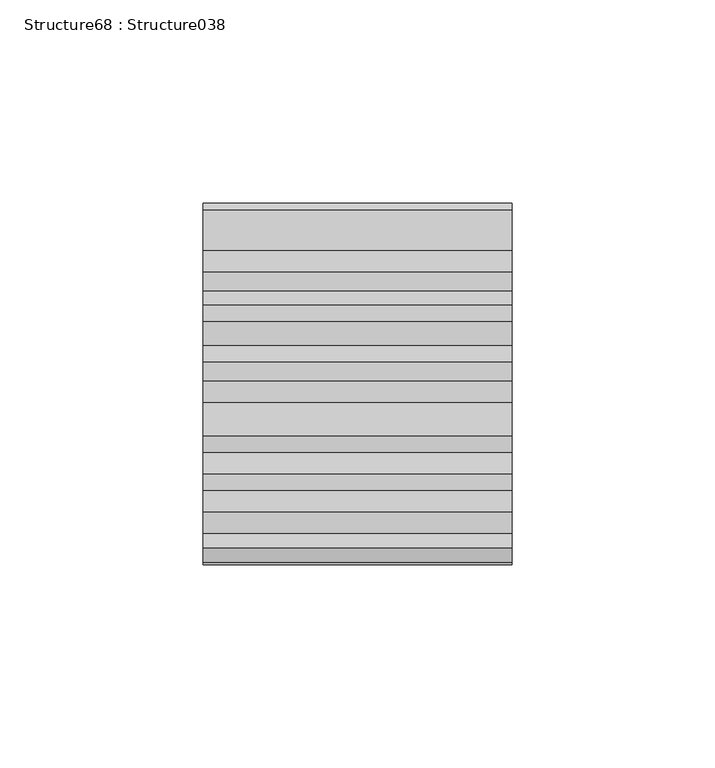
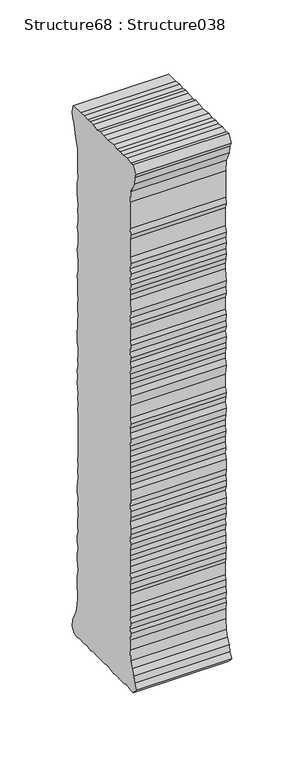
"""IFC4 building model written with IfcOpenShell, lengths in millimetres: proxy geometry, Structure68 : Structure038."""

from ifc_helpers import new_model, si_unit, frame, origin, place, context, project, spatial, polyline, outline, extrude, source, transform, mapped, element, save


def structure68_structure038_898fa140(model_context):
    return source(origin(), model_context, "Body", "SweptSolid", [
        extrude(outline(polyline([(279690.2824701, 3575.6853037), (279690.8761737, 3583.8864372), (279690.8761737, 3592.6700423), (279690.2824701, 3598.5284533), (279690.8761737, 3602.0280957), (279690.2824701, 3606.7295868), (279690.8761737, 3611.4134274), (279690.8761737, 3617.2718384), (279691.4586452, 3620.7971545), (279691.4586452, 3631.3410106), (279690.8761737, 3634.856699), (279690.8761737, 3640.114988), (279690.2824701, 3644.8245022), (279690.8761737, 3648.9258713), (279690.8761737, 3654.7842823), (279691.4586452, 3659.4584952), (279690.8761737, 3664.1423357), (279691.4586452, 3668.2437048), (279690.2824701, 3673.5276674), (279690.8761737, 3678.2018803), (279690.2824701, 3682.3289231), (279690.2824701, 3687.0127636), (279691.4586452, 3692.2710525), (279690.2824701, 3696.3884676), (279690.2824701, 3701.6547796), (279690.8761737, 3705.7545441), (279690.2824701, 3711.0304837), (279690.2824701, 3719.2316172), (279691.4586452, 3723.9154578), (279690.8761737, 3728.5992983), (279691.4586452, 3733.2991849), (279691.4586452, 3737.9750024), (279690.8761737, 3742.6748889), (279691.4586452, 3747.3587295), (279691.4586452, 3752.04257), (279690.8761737, 3756.7440611), (279690.2824701, 3762.5848215), (279691.4586452, 3767.2590344), (279690.8761737, 3771.9605256), (279690.2824701, 3775.4874463), (279691.4586452, 3780.1616592), (279691.4586452, 3790.7039107), (279690.2824701, 3798.9050443), (279691.4586452, 3804.1890069), (279691.4586452, 3808.8888934), (279690.8761737, 3813.5743386), (279690.8761737, 3817.6741031), (279690.2824701, 3822.932392), (279691.4586452, 3827.6162325), (279690.2824701, 3831.732043), (279690.8761737, 3836.4174882), (279690.2824701, 3842.2758992), (279691.4586452, 3845.8012153), (279691.4586452, 3855.7353217), (279690.2824701, 3859.8591552), (279690.8761737, 3865.1190488), (279690.2824701, 3870.4030114), (279691.4586452, 3879.7610648), (279691.4586452, 3884.4609514), (279690.8761737, 3888.5623205), (279690.2824701, 3893.246161), (279690.8761737, 3897.3475301), (279690.2824701, 3902.6314927), (279690.8761737, 3906.7328618), (279690.2824701, 3911.4054701), (279691.4586452, 3916.0909152), (279691.4586452, 3931.3346579), (279690.2824701, 3935.4328178), (279690.8761737, 3940.718385), (279690.8761737, 3962.9774586), (279690.2824701, 3972.3627903), (279685.6098618, 3981.7208437), (279685.0161581, 3987.5792547), (279683.2575116, 3991.0788971), (279686.765177, 3997.5486624), (279690.2824701, 3996.390138), (279695.5584096, 3997.5486624), (279700.8359538, 3996.9645864), (279704.9341137, 3997.5486624), (279710.2116579, 3996.390138), (279714.3114224, 3997.5486624), (279722.5189744, 3996.390138), (279727.7852863, 3996.9645864), (279732.4787545, 3997.5486624), (279736.5801236, 3996.390138), (279742.4305116, 3997.5486624), (279746.5366945, 3997.5486624), (279750.0475691, 3996.9645864), (279754.7394327, 3997.5486624), (279760.0137676, 3996.9645864), (279769.9735477, 3996.9645864), (279771.7321943, 3991.0788971), (279770.5656468, 3986.4046842), (279768.7989772, 3982.3225704), (279768.2245288, 3978.2035506), (279766.4562547, 3972.3627903), (279764.1151367, 3964.1343784), (279764.1151367, 3944.8165449), (279763.5310607, 3939.5325823), (279764.6992128, 3935.4328178), (279764.6992128, 3925.4746423), (279764.1151367, 3921.3748778), (279763.5310607, 3916.6653636), (279764.1151367, 3911.4054701), (279763.5310607, 3907.888177), (279763.5310607, 3903.2059411), (279764.6992128, 3897.3475301), (279763.5310607, 3893.246161), (279763.5310607, 3883.8881076), (279764.6992128, 3878.5784713), (279764.1151367, 3874.5043805), (279763.5310607, 3869.2444869), (279763.5310607, 3861.0192843), (279764.6992128, 3856.3161885), (279764.1151367, 3851.6612309), (279764.1151367, 3841.0900965), (279763.5310607, 3836.9919366), (279764.1151367, 3832.8921721), (279764.1151367, 3828.2163546), (279763.5310607, 3822.932392), (279764.1151367, 3818.8310229), (279764.1151367, 3812.9726119), (279764.6992128, 3808.8888934), (279764.6992128, 3800.0876378), (279763.5310607, 3795.4037973), (279763.5310607, 3790.7039107), (279764.1151367, 3785.4456218), (279763.5310607, 3781.3282066), (279764.6992128, 3776.0618947), (279764.1151367, 3770.8036057), (279764.6992128, 3766.1021146), (279764.1151367, 3762.0023501), (279763.5310607, 3756.7440611), (279764.1151367, 3753.2171405), (279763.5310607, 3748.5429276), (279764.1151367, 3742.6748889), (279763.5310607, 3739.1592005), (279763.5310607, 3705.7545441), (279764.1151367, 3700.4705815), (279763.5310607, 3696.3884676), (279764.1151367, 3691.0868544), (279763.5310607, 3686.4030139), (279764.1151367, 3681.7271964), (279764.6992128, 3677.6274319), (279764.6992128, 3673.5276674), (279763.5310607, 3668.8261762), (279764.1151367, 3663.5598643), (279763.5310607, 3658.8840468), (279763.5310607, 3654.1841602), (279764.1151367, 3649.5003197), (279764.1151367, 3644.2420307), (279763.5310607, 3640.114988), (279764.6992128, 3636.0408972), (279764.6992128, 3631.3410106), (279763.5310607, 3626.6571701), (279764.6992128, 3620.7971545), (279764.6992128, 3616.69739), (279764.1151367, 3612.5976255), (279763.5310607, 3607.3393366), (279764.6992128, 3602.0280957), (279764.6992128, 3592.6700423), (279764.1151367, 3587.9685511), (279764.1151367, 3583.2863152), (279765.2816842, 3573.9266571), (279767.0499583, 3569.8268927), (279768.7989772, 3565.7094775), (279771.1481182, 3561.025637), (279771.7321943, 3555.1848766), (279768.7989772, 3551.0658569), (279765.2816842, 3550.4833855), (279760.6074713, 3551.0658569), (279754.7394327, 3551.0658569), (279751.2221396, 3551.6675836), (279745.9462, 3550.4833855), (279742.4305116, 3551.6675836), (279737.7546941, 3551.0658569), (279727.1947919, 3551.0658569), (279722.5189744, 3551.6675836), (279718.4095823, 3551.0658569), (279713.7273464, 3550.4833855), (279709.6179542, 3551.0658569), (279704.9341137, 3550.4833855), (279699.6678018, 3550.4833855), (279696.1505087, 3551.6675836), (279690.8761737, 3550.4833855), (279686.765177, 3550.4833855), (279682.6654125, 3555.1848766), (279685.0161581, 3559.8671125), (279686.1827056, 3565.1254015), (279688.5334512, 3569.8268927), (279690.2824701, 3575.6853037)])), frame((-59031.6926606, 0.0, 0.0), z_axis=(1.0, 0.0, 0.0), x_axis=(0.0, 1.0, 0.0)), (0.0, 0.0, 1.0), 76.2),
    ])


if __name__ == "__main__":
    model = new_model("IFC4")
    model_context = context("Model", 3, world=origin())
    ifc_project = project(units=[si_unit("LENGTHUNIT", "METRE", prefix="MILLI")], contexts=[model_context])
    site = spatial("IfcSite", under=ifc_project)
    building = spatial("IfcBuilding", under=site)
    placement = place(None, origin())
    structure68_structure038_shape = structure68_structure038_898fa140(model_context)
    element("IfcBuildingElementProxy", 1, Name="Structure68 : Structure038", ObjectType="Structure68 : Structure038", at=placement, inside=building, context=model_context, shape_type="MappedRepresentation", body=[
        mapped(structure68_structure038_shape, transform((0.0, 0.0, 0.0), x_axis=(1.0, 0.0, 0.0), y_axis=(0.0, 1.0, 0.0), z_axis=(0.0, 0.0, 1.0))),
    ])
    save(model, "model.ifc")

# Revit data of these elements
# Type "Structure68 : Structure038"
#   NameOverride = "Structure038"
# Element 1 (IfcBuildingElementProxy, "Structure68 : Structure038")
#   Materials on its faces: "BRUSHED ALUM. LETTERING"
# Materials
#   "BRUSHED ALUM. LETTERING": class "Unassigned", colour RGB 169 181 186, transparency 0, Cost = 0
